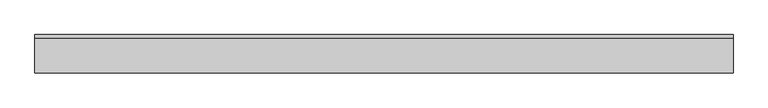
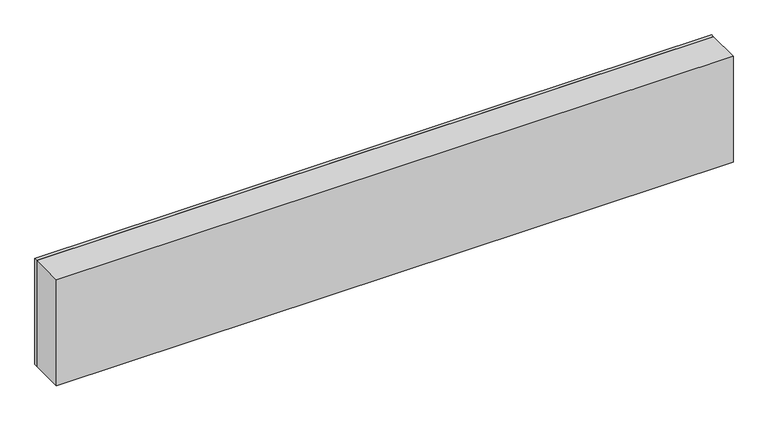
"""IFC4 building model written with IfcOpenShell, lengths in millimetres: furniture geometry, OD_CW_Upper Cabinet : OD_CW_Upper Cabinet."""

import ifcopenshell
import ifcopenshell.guid

model = None  # the IFC model being written
_history = None  # IfcOwnerHistory: only IFC2X3 demands one
_inside = {}  # id of a spatial element -> (the spatial element, [elements in it])
_under = {}  # id of a project, library or spatial element -> (it, [spatial elements below it])
_declared = {}  # id of a project -> (the project, [libraries it declares])
_typed = {}  # id of a type object -> (the type object, [elements of that type])
_made_of = {}  # id of a material, layer set ... -> (it, [elements and type objects made of it])


def new_model(schema):
    """Start an empty IFC model of exactly this schema.

    Asked for "IFC4X3", IfcOpenShell would pick the latest addendum, in which some entities
    have other attributes; the version numbers below select the first issue.
    IFC2X3 requires an IfcOwnerHistory on every rooted entity: one is made here for all.
    """
    global model, _history
    if schema == "IFC4X3":
        model = ifcopenshell.file(schema_version=(4, 3, 0, 0))
    else:
        model = ifcopenshell.file(schema=schema)
    _inside.clear()
    _under.clear()
    _declared.clear()
    _typed.clear()
    _made_of.clear()
    _history = None
    if model.schema == "IFC2X3":
        org = make("IfcOrganization", Name="unknown")
        user = make(
            "IfcPersonAndOrganization",
            ThePerson=make("IfcPerson", FamilyName="unknown"),
            TheOrganization=org,
        )
        app = make(
            "IfcApplication",
            ApplicationDeveloper=org,
            Version="unknown",
            ApplicationFullName="unknown",
            ApplicationIdentifier="unknown",
        )
        _history = make(
            "IfcOwnerHistory",
            OwningUser=user,
            OwningApplication=app,
            ChangeAction="ADDED",
            CreationDate=0,
        )
    return model


def make(cls, **values):
    """One entity of the class cls with the attributes given. An attribute that is None is left unset."""
    return model.create_entity(
        cls, **{name: value for name, value in values.items() if value is not None}
    )


def rooted(cls, **values):
    """An entity with a GlobalId (a new one), such as an element, a storey or a relation."""
    return make(cls, GlobalId=ifcopenshell.guid.new(), OwnerHistory=_history, **values)


def si_unit(unit_type, name, prefix=None):
    """IfcSIUnit, for example si_unit("LENGTHUNIT", "METRE", prefix="MILLI")."""
    return make("IfcSIUnit", UnitType=unit_type, Prefix=prefix, Name=name)


def assignment(units):
    """IfcUnitAssignment: the units of a project."""
    return None if units is None else make("IfcUnitAssignment", Units=units)


def point(xyz):
    """IfcCartesianPoint."""
    return None if xyz is None else make("IfcCartesianPoint", Coordinates=xyz)


def direction(xyz):
    """IfcDirection."""
    return None if xyz is None else make("IfcDirection", DirectionRatios=xyz)


def frame(location, z_axis=None, x_axis=None):
    """IfcAxis2Placement3D, a coordinate frame: its origin and axes. An axis left out is left unset."""
    return make(
        "IfcAxis2Placement3D",
        Location=point(location),
        Axis=direction(z_axis),
        RefDirection=direction(x_axis),
    )


def origin():
    """The frame at (0, 0, 0) with its axes left unset."""
    return frame((0.0, 0.0, 0.0))


def place(relative_to, where):
    """IfcLocalPlacement: puts the frame where relative to a parent placement (None: the world)."""
    return make(
        "IfcLocalPlacement", PlacementRelTo=relative_to, RelativePlacement=where
    )


def context(
    kind, dimensions, precision=None, world=None, true_north=None, identifier=None
):
    """IfcGeometricRepresentationContext, for example the 3D "Model" context."""
    return make(
        "IfcGeometricRepresentationContext",
        ContextIdentifier=identifier,
        ContextType=kind,
        CoordinateSpaceDimension=dimensions,
        Precision=precision,
        WorldCoordinateSystem=world,
        TrueNorth=true_north,
    )


def project(units=None, contexts=None):
    """IfcProject with its units and contexts."""
    return rooted(
        "IfcProject",
        Name="project",
        RepresentationContexts=contexts,
        UnitsInContext=assignment(units),
    )


def spatial(cls, under=None, at=None, **own):
    """A site, building, storey or space (cls), placed at a placement, below another one or the project."""
    s = rooted(cls, ObjectPlacement=at, **own)
    if under is not None:
        _under.setdefault(under.id(), (under, []))[1].append(s)
    return s


def polyline(points):
    """IfcPolyline through the points."""
    return make("IfcPolyline", Points=[point(p) for p in points])


def outline(outer, holes=None, kind="AREA"):
    """IfcArbitraryClosedProfileDef: a profile drawn as a closed curve; with holes, ...WithVoids."""
    if holes is None:
        return make("IfcArbitraryClosedProfileDef", ProfileType=kind, OuterCurve=outer)
    return make(
        "IfcArbitraryProfileDefWithVoids",
        ProfileType=kind,
        OuterCurve=outer,
        InnerCurves=holes,
    )


def extrude(swept, where, along, depth):
    """IfcExtrudedAreaSolid: the profile swept, set in the frame where, extruded along a direction by depth."""
    return make(
        "IfcExtrudedAreaSolid",
        SweptArea=swept,
        Position=where,
        ExtrudedDirection=direction(along),
        Depth=depth,
    )


def shape(context_of_items, identifier, shape_type, items):
    """IfcShapeRepresentation: the items that make up one representation, for example the "Body"."""
    return make(
        "IfcShapeRepresentation",
        ContextOfItems=context_of_items,
        RepresentationIdentifier=identifier,
        RepresentationType=shape_type,
        Items=items,
    )


def source(mapping_origin, context_of_items, identifier, shape_type, items):
    """IfcRepresentationMap: a shape defined once, which mapped items show again and again."""
    return make(
        "IfcRepresentationMap",
        MappingOrigin=mapping_origin,
        MappedRepresentation=shape(context_of_items, identifier, shape_type, items),
    )


def transform(
    local_origin,
    x_axis=None,
    y_axis=None,
    z_axis=None,
    scale=None,
    scale2=None,
    scale3=None,
    uniform=True,
):
    """IfcCartesianTransformationOperator3D, or its non-uniform kind. x_axis, y_axis, z_axis: its Axis1, 2, 3."""
    if uniform:
        return make(
            "IfcCartesianTransformationOperator3D",
            Axis1=direction(x_axis),
            Axis2=direction(y_axis),
            LocalOrigin=point(local_origin),
            Scale=scale,
            Axis3=direction(z_axis),
        )
    return make(
        "IfcCartesianTransformationOperator3DnonUniform",
        Axis1=direction(x_axis),
        Axis2=direction(y_axis),
        LocalOrigin=point(local_origin),
        Scale=scale,
        Axis3=direction(z_axis),
        Scale2=scale2,
        Scale3=scale3,
    )


def mapped(mapping_source, mapping_target):
    """IfcMappedItem: shows the shape of a source again, moved by a transform."""
    return make(
        "IfcMappedItem", MappingSource=mapping_source, MappingTarget=mapping_target
    )


def made_of(thing, what):
    """Note that an element or type object is made of a material, layer set ...; save() writes the relation."""
    if what is not None:
        _made_of.setdefault(what.id(), (what, []))[1].append(thing)
    return thing


def element(
    cls,
    number,
    at=None,
    inside=None,
    cuts=None,
    type_object=None,
    material=None,
    context=None,
    identifier="Body",
    shape_type=None,
    held_by="IfcProductDefinitionShape",
    body=None,
    shapes=None,
    **own,
):
    """One element of the class cls, such as IfcWall. Its Tag is "e" and its number.

    at: its placement. inside: the storey or other place that contains it. cuts: it is an
    opening in that element (IfcRelVoidsElement). A single representation is given by context,
    identifier, shape_type and body (its items); several are given by shapes. held_by: the class
    of the entity that holds the representations. save() writes the other relations.
    """
    e = rooted(cls, Tag="e%d" % number, ObjectPlacement=at, **own)
    if body is not None:
        shapes = [shape(context, identifier, shape_type, body)]
    if shapes is not None:
        e.Representation = make(held_by, Representations=shapes)
    if inside is not None:
        _inside.setdefault(inside.id(), (inside, []))[1].append(e)
    if cuts is not None:
        rooted(
            "IfcRelVoidsElement", RelatingBuildingElement=cuts, RelatedOpeningElement=e
        )
    if type_object is not None:
        _typed.setdefault(type_object.id(), (type_object, []))[1].append(e)
    return made_of(e, material)


def aggregate(whole, parts):
    """IfcRelAggregates: a whole, such as a stair, and the parts it consists of."""
    return rooted("IfcRelAggregates", RelatingObject=whole, RelatedObjects=parts)


def save(model, path):
    """Write the relations noted so far, then the file.

    IfcRelAggregates (storeys below a building ...), IfcRelContainedInSpatialStructure (elements
    in a storey), IfcRelDefinesByType, IfcRelAssociatesMaterial and IfcRelDeclares: one each for
    every whole, place, type object, material and project.
    """
    for whole, parts in _under.values():
        aggregate(whole, parts)
    for where, things in _inside.values():
        rooted(
            "IfcRelContainedInSpatialStructure",
            RelatedElements=things,
            RelatingStructure=where,
        )
    for kind, things in _typed.values():
        rooted("IfcRelDefinesByType", RelatedObjects=things, RelatingType=kind)
    for what, things in _made_of.values():
        rooted("IfcRelAssociatesMaterial", RelatedObjects=things, RelatingMaterial=what)
    for by, libraries in _declared.values():
        rooted("IfcRelDeclares", RelatingContext=by, RelatedDefinitions=libraries)
    model.write(path)


def furniture_9815a7d2(model_context):
    return source(origin(), model_context, "Body", "SweptSolid", [
        extrude(outline(polyline([(18.7377049, -330.2), (18.7377049, -304.8), (5543.8678379, -304.8), (5543.8678379, -330.2), (18.7377049, -330.2)])), frame((0.0, 0.0, 965.2), z_axis=(0.0, 0.0, 1.0), x_axis=(1.0, 0.0, 0.0)), (0.0, 0.0, 1.0), 914.4),
        extrude(outline(polyline([(18.7377049, -609.6), (18.7377049, -330.2), (5543.8678379, -330.2), (5543.8678379, -609.6), (18.7377049, -609.6)])), frame((0.0, 0.0, 965.2), z_axis=(0.0, 0.0, 1.0), x_axis=(1.0, 0.0, 0.0)), (0.0, 0.0, 1.0), 914.4),
    ])


if __name__ == "__main__":
    model = new_model("IFC4")
    model_context = context("Model", 3, world=origin())
    ifc_project = project(units=[si_unit("LENGTHUNIT", "METRE", prefix="MILLI")], contexts=[model_context])
    site = spatial("IfcSite", under=ifc_project)
    building = spatial("IfcBuilding", under=site)
    placement = place(None, origin())
    furniture_shape = furniture_9815a7d2(model_context)
    element("IfcFurniture", 1, ObjectType="OD_CW_Upper Cabinet : OD_CW_Upper Cabinet", at=placement, inside=building, context=model_context, shape_type="MappedRepresentation", body=[
        mapped(furniture_shape, transform((0.0, 0.0, 0.0), x_axis=(1.0, 0.0, 0.0), y_axis=(0.0, 1.0, 0.0), z_axis=(0.0, 0.0, 1.0))),
    ])
    save(model, "model.ifc")

# Revit data of these elements
# Type "OD_CW_Upper Cabinet : OD_CW_Upper Cabinet"
#   OD_CW_Width [instance default] = 2' - 2"
#   OD_CW_Off Floor [instance default] = 3' - 2"
#   OD_CW_Length [instance default] = 8' - 0"
#   OD_CW_Height [instance default] = 7' - 0"
#   Depth = 2' - 0"
#   Height = 3' - 0"
#   Width = 4' - 0"
#   OD_CW_Material_Front Panel [instance default] = none
# Element 1 (IfcFurniture, "OD_CW_Upper Cabinet : OD_CW_Upper Cabinet")
#   OD_CW_Width = 1' - 0"
#   OD_CW_Length = 18' - 1.52481"
#   OD_CW_Height = 3' - 0"
